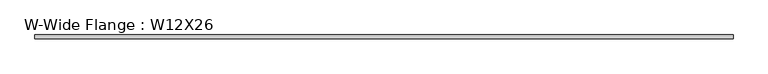
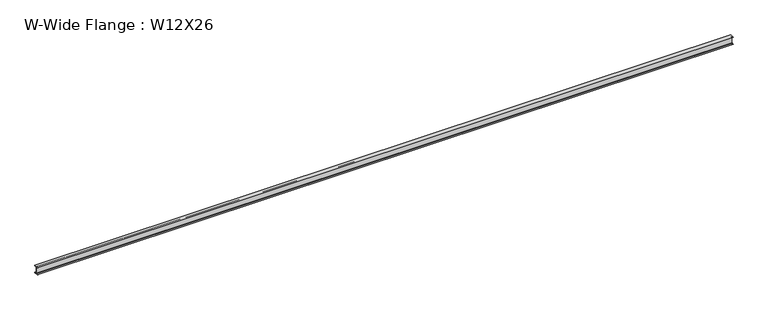
"""IFC4 building model written with IfcOpenShell, lengths in millimetres: beam geometry, W-Wide Flange : W12X26."""

import ifcopenshell
import ifcopenshell.guid

model = None  # the IFC model being written
_history = None  # IfcOwnerHistory: only IFC2X3 demands one
_inside = {}  # id of a spatial element -> (the spatial element, [elements in it])
_under = {}  # id of a project, library or spatial element -> (it, [spatial elements below it])
_declared = {}  # id of a project -> (the project, [libraries it declares])
_typed = {}  # id of a type object -> (the type object, [elements of that type])
_made_of = {}  # id of a material, layer set ... -> (it, [elements and type objects made of it])


def new_model(schema):
    """Start an empty IFC model of exactly this schema.

    Asked for "IFC4X3", IfcOpenShell would pick the latest addendum, in which some entities
    have other attributes; the version numbers below select the first issue.
    IFC2X3 requires an IfcOwnerHistory on every rooted entity: one is made here for all.
    """
    global model, _history
    if schema == "IFC4X3":
        model = ifcopenshell.file(schema_version=(4, 3, 0, 0))
    else:
        model = ifcopenshell.file(schema=schema)
    _inside.clear()
    _under.clear()
    _declared.clear()
    _typed.clear()
    _made_of.clear()
    _history = None
    if model.schema == "IFC2X3":
        org = make("IfcOrganization", Name="unknown")
        user = make(
            "IfcPersonAndOrganization",
            ThePerson=make("IfcPerson", FamilyName="unknown"),
            TheOrganization=org,
        )
        app = make(
            "IfcApplication",
            ApplicationDeveloper=org,
            Version="unknown",
            ApplicationFullName="unknown",
            ApplicationIdentifier="unknown",
        )
        _history = make(
            "IfcOwnerHistory",
            OwningUser=user,
            OwningApplication=app,
            ChangeAction="ADDED",
            CreationDate=0,
        )
    return model


def make(cls, **values):
    """One entity of the class cls with the attributes given. An attribute that is None is left unset."""
    return model.create_entity(
        cls, **{name: value for name, value in values.items() if value is not None}
    )


def rooted(cls, **values):
    """An entity with a GlobalId (a new one), such as an element, a storey or a relation."""
    return make(cls, GlobalId=ifcopenshell.guid.new(), OwnerHistory=_history, **values)


def si_unit(unit_type, name, prefix=None):
    """IfcSIUnit, for example si_unit("LENGTHUNIT", "METRE", prefix="MILLI")."""
    return make("IfcSIUnit", UnitType=unit_type, Prefix=prefix, Name=name)


def assignment(units):
    """IfcUnitAssignment: the units of a project."""
    return None if units is None else make("IfcUnitAssignment", Units=units)


def point(xyz):
    """IfcCartesianPoint."""
    return None if xyz is None else make("IfcCartesianPoint", Coordinates=xyz)


def direction(xyz):
    """IfcDirection."""
    return None if xyz is None else make("IfcDirection", DirectionRatios=xyz)


def frame(location, z_axis=None, x_axis=None):
    """IfcAxis2Placement3D, a coordinate frame: its origin and axes. An axis left out is left unset."""
    return make(
        "IfcAxis2Placement3D",
        Location=point(location),
        Axis=direction(z_axis),
        RefDirection=direction(x_axis),
    )


def frame_2d(location, x_axis=None):
    """IfcAxis2Placement2D, a coordinate frame in the plane: its origin and x axis."""
    return make(
        "IfcAxis2Placement2D", Location=point(location), RefDirection=direction(x_axis)
    )


def origin():
    """The frame at (0, 0, 0) with its axes left unset."""
    return frame((0.0, 0.0, 0.0))


def place(relative_to, where):
    """IfcLocalPlacement: puts the frame where relative to a parent placement (None: the world)."""
    return make(
        "IfcLocalPlacement", PlacementRelTo=relative_to, RelativePlacement=where
    )


def context(
    kind, dimensions, precision=None, world=None, true_north=None, identifier=None
):
    """IfcGeometricRepresentationContext, for example the 3D "Model" context."""
    return make(
        "IfcGeometricRepresentationContext",
        ContextIdentifier=identifier,
        ContextType=kind,
        CoordinateSpaceDimension=dimensions,
        Precision=precision,
        WorldCoordinateSystem=world,
        TrueNorth=true_north,
    )


def project(units=None, contexts=None):
    """IfcProject with its units and contexts."""
    return rooted(
        "IfcProject",
        Name="project",
        RepresentationContexts=contexts,
        UnitsInContext=assignment(units),
    )


def spatial(cls, under=None, at=None, **own):
    """A site, building, storey or space (cls), placed at a placement, below another one or the project."""
    s = rooted(cls, ObjectPlacement=at, **own)
    if under is not None:
        _under.setdefault(under.id(), (under, []))[1].append(s)
    return s


def polyline(points):
    """IfcPolyline through the points."""
    return make("IfcPolyline", Points=[point(p) for p in points])


def circle_curve(where, radius):
    """IfcCircle in the frame where."""
    return make("IfcCircle", Position=where, Radius=radius)


def trimmed(basis, trim1, trim2, sense, master):
    """IfcTrimmedCurve: the piece of a basis curve between two trims."""
    return make(
        "IfcTrimmedCurve",
        BasisCurve=basis,
        Trim1=trim1,
        Trim2=trim2,
        SenseAgreement=sense,
        MasterRepresentation=master,
    )


def segment(curve, same_sense, transition):
    """IfcCompositeCurveSegment."""
    return make(
        "IfcCompositeCurveSegment",
        Transition=transition,
        SameSense=same_sense,
        ParentCurve=curve,
    )


def composite_curve(segments, self_intersect=None):
    """IfcCompositeCurve: segments joined end to end."""
    return make("IfcCompositeCurve", Segments=segments, SelfIntersect=self_intersect)


def outline(outer, holes=None, kind="AREA"):
    """IfcArbitraryClosedProfileDef: a profile drawn as a closed curve; with holes, ...WithVoids."""
    if holes is None:
        return make("IfcArbitraryClosedProfileDef", ProfileType=kind, OuterCurve=outer)
    return make(
        "IfcArbitraryProfileDefWithVoids",
        ProfileType=kind,
        OuterCurve=outer,
        InnerCurves=holes,
    )


def extrude(swept, where, along, depth):
    """IfcExtrudedAreaSolid: the profile swept, set in the frame where, extruded along a direction by depth."""
    return make(
        "IfcExtrudedAreaSolid",
        SweptArea=swept,
        Position=where,
        ExtrudedDirection=direction(along),
        Depth=depth,
    )


def shape(context_of_items, identifier, shape_type, items):
    """IfcShapeRepresentation: the items that make up one representation, for example the "Body"."""
    return make(
        "IfcShapeRepresentation",
        ContextOfItems=context_of_items,
        RepresentationIdentifier=identifier,
        RepresentationType=shape_type,
        Items=items,
    )


def source(mapping_origin, context_of_items, identifier, shape_type, items):
    """IfcRepresentationMap: a shape defined once, which mapped items show again and again."""
    return make(
        "IfcRepresentationMap",
        MappingOrigin=mapping_origin,
        MappedRepresentation=shape(context_of_items, identifier, shape_type, items),
    )


def transform(
    local_origin,
    x_axis=None,
    y_axis=None,
    z_axis=None,
    scale=None,
    scale2=None,
    scale3=None,
    uniform=True,
):
    """IfcCartesianTransformationOperator3D, or its non-uniform kind. x_axis, y_axis, z_axis: its Axis1, 2, 3."""
    if uniform:
        return make(
            "IfcCartesianTransformationOperator3D",
            Axis1=direction(x_axis),
            Axis2=direction(y_axis),
            LocalOrigin=point(local_origin),
            Scale=scale,
            Axis3=direction(z_axis),
        )
    return make(
        "IfcCartesianTransformationOperator3DnonUniform",
        Axis1=direction(x_axis),
        Axis2=direction(y_axis),
        LocalOrigin=point(local_origin),
        Scale=scale,
        Axis3=direction(z_axis),
        Scale2=scale2,
        Scale3=scale3,
    )


def mapped(mapping_source, mapping_target):
    """IfcMappedItem: shows the shape of a source again, moved by a transform."""
    return make(
        "IfcMappedItem", MappingSource=mapping_source, MappingTarget=mapping_target
    )


def made_of(thing, what):
    """Note that an element or type object is made of a material, layer set ...; save() writes the relation."""
    if what is not None:
        _made_of.setdefault(what.id(), (what, []))[1].append(thing)
    return thing


def element(
    cls,
    number,
    at=None,
    inside=None,
    cuts=None,
    type_object=None,
    material=None,
    context=None,
    identifier="Body",
    shape_type=None,
    held_by="IfcProductDefinitionShape",
    body=None,
    shapes=None,
    **own,
):
    """One element of the class cls, such as IfcWall. Its Tag is "e" and its number.

    at: its placement. inside: the storey or other place that contains it. cuts: it is an
    opening in that element (IfcRelVoidsElement). A single representation is given by context,
    identifier, shape_type and body (its items); several are given by shapes. held_by: the class
    of the entity that holds the representations. save() writes the other relations.
    """
    e = rooted(cls, Tag="e%d" % number, ObjectPlacement=at, **own)
    if body is not None:
        shapes = [shape(context, identifier, shape_type, body)]
    if shapes is not None:
        e.Representation = make(held_by, Representations=shapes)
    if inside is not None:
        _inside.setdefault(inside.id(), (inside, []))[1].append(e)
    if cuts is not None:
        rooted(
            "IfcRelVoidsElement", RelatingBuildingElement=cuts, RelatedOpeningElement=e
        )
    if type_object is not None:
        _typed.setdefault(type_object.id(), (type_object, []))[1].append(e)
    return made_of(e, material)


def aggregate(whole, parts):
    """IfcRelAggregates: a whole, such as a stair, and the parts it consists of."""
    return rooted("IfcRelAggregates", RelatingObject=whole, RelatedObjects=parts)


def save(model, path):
    """Write the relations noted so far, then the file.

    IfcRelAggregates (storeys below a building ...), IfcRelContainedInSpatialStructure (elements
    in a storey), IfcRelDefinesByType, IfcRelAssociatesMaterial and IfcRelDeclares: one each for
    every whole, place, type object, material and project.
    """
    for whole, parts in _under.values():
        aggregate(whole, parts)
    for where, things in _inside.values():
        rooted(
            "IfcRelContainedInSpatialStructure",
            RelatedElements=things,
            RelatingStructure=where,
        )
    for kind, things in _typed.values():
        rooted("IfcRelDefinesByType", RelatedObjects=things, RelatingType=kind)
    for what, things in _made_of.values():
        rooted("IfcRelAssociatesMaterial", RelatedObjects=things, RelatingMaterial=what)
    for by, libraries in _declared.values():
        rooted("IfcRelDeclares", RelatingContext=by, RelatedDefinitions=libraries)
    model.write(path)


def w_wide_flange_w12x26_db84f3f3(model_context):
    return source(origin(), model_context, "Body", "SweptSolid", [
        extrude(outline(composite_curve([segment(polyline([(82.4011719, -145.5539063), (82.4011719, -155.178125), (-82.4011719, -155.178125), (-82.4011719, -145.5539063), (-20.2902344, -145.5539063)]), True, "CONTINUOUS"), segment(trimmed(circle_curve(frame_2d((-20.2902344, -128.190625)), 17.3632812), [point((-20.2902344, -145.5539063))], [point((-2.9269531, -128.190625))], True, "CARTESIAN"), True, "CONTINUOUS"), segment(polyline([(-2.9269531, -128.190625), (-2.9269531, 128.190625)]), True, "CONTINUOUS"), segment(trimmed(circle_curve(frame_2d((-20.2902344, 128.190625)), 17.3632812), [point((-2.9269531, 128.190625))], [point((-20.2902344, 145.5539062))], True, "CARTESIAN"), True, "CONTINUOUS"), segment(polyline([(-20.2902344, 145.5539062), (-82.4011719, 145.5539062), (-82.4011719, 155.178125), (82.4011719, 155.178125), (82.4011719, 145.5539062), (20.2902344, 145.5539062)]), True, "CONTINUOUS"), segment(trimmed(circle_curve(frame_2d((20.2902344, 128.190625)), 17.3632812), [point((20.2902344, 145.5539062))], [point((2.9269531, 128.190625))], True, "CARTESIAN"), True, "CONTINUOUS"), segment(polyline([(2.9269531, 128.190625), (2.9269531, -128.190625)]), True, "CONTINUOUS"), segment(trimmed(circle_curve(frame_2d((20.2902344, -128.190625)), 17.3632812), [point((2.9269531, -128.190625))], [point((20.2902344, -145.5539063))], True, "CARTESIAN"), True, "CONTINUOUS"), segment(polyline([(20.2902344, -145.5539063), (82.4011719, -145.5539063)]), True, "CONTINUOUS")], self_intersect=False)), frame((-14249.4, 0.0, 0.0), z_axis=(1.0, 0.0, 0.0), x_axis=(0.0, 1.0, 0.0)), (0.0, 0.0, 1.0), 28498.8),
    ])


if __name__ == "__main__":
    model = new_model("IFC4")
    model_context = context("Model", 3, world=origin())
    ifc_project = project(units=[si_unit("LENGTHUNIT", "METRE", prefix="MILLI")], contexts=[model_context])
    site = spatial("IfcSite", under=ifc_project)
    building = spatial("IfcBuilding", under=site)
    placement = place(None, origin())
    w_wide_flange_w12x26_shape = w_wide_flange_w12x26_db84f3f3(model_context)
    element("IfcBeam", 1, ObjectType="W-Wide Flange : W12X26", at=placement, inside=building, context=model_context, shape_type="MappedRepresentation", body=[
        mapped(w_wide_flange_w12x26_shape, transform((0.0, 0.0, 0.0), x_axis=(1.0, 0.0, 0.0), y_axis=(0.0, 1.0, 0.0), z_axis=(0.0, 0.0, 1.0))),
    ])
    save(model, "model.ifc")

# Revit data of these elements
# Type "W-Wide Flange : W12X26"
#   Assembly Code = "B10"
#   W = 26
#   Length [instance default] = 5' - 0"
#   bf = 0' - 6 125/256"
#   d = 1' - 0 7/32"
#   k = 0' - 1 1/16"
#   k2 = 0' - 0 175/256"
#   tf = 0' - 0 97/256"
#   tw = 0' - 0 59/256"
#   A = 0.053125 SF
#   Structural Material [instance default] = none
